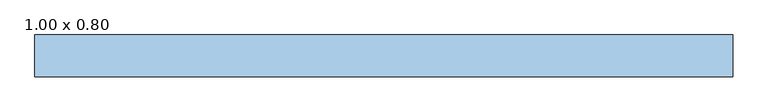
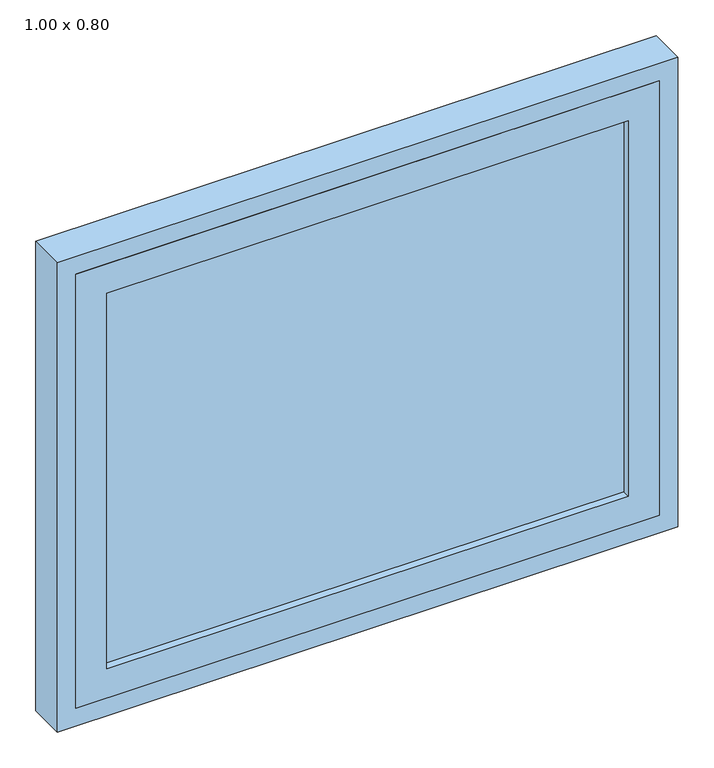
"""IFC4 building model written with IfcOpenShell, lengths in millimetres: window geometry, CC_JANELA MAXIM-AR_1 FOLHA VIDRO : 1.00 x 0.80."""

from ifc_helpers import new_model, si_unit, frame, origin, place, context, project, spatial, polyline, outline, extrude, source, transform, mapped, element, save


def window_1_00_x_0_80_3e14d2bc(model_context):
    return source(origin(), model_context, "Body", "SweptSolid", [
        extrude(outline(polyline([(-420.0, -87.5), (-420.0, -82.5), (420.0, -82.5), (420.0, -87.5), (-420.0, -87.5)])), frame((0.0, 0.0, 1780.0), z_axis=(0.0, 0.0, 1.0), x_axis=(1.0, 0.0, 0.0)), (0.0, 0.0, 1.0), 640.0),
        extrude(outline(polyline([(2470.0, -470.0), (1730.0, -470.0), (1730.0, 470.0), (2470.0, 470.0), (2470.0, -470.0)]), holes=[polyline([(2420.0, 420.0), (1780.0, 420.0), (1780.0, -420.0), (2420.0, -420.0), (2420.0, 420.0)])]), frame((0.0, -100.0, 0.0), z_axis=(0.0, 1.0, 0.0), x_axis=(0.0, 0.0, 1.0)), (0.0, 0.0, 1.0), 30.0),
        extrude(outline(polyline([(1700.0, 500.0), (2500.0, 500.0), (2500.0, -500.0), (1700.0, -500.0), (1700.0, 500.0)]), holes=[polyline([(1730.0, -470.0), (2470.0, -470.0), (2470.0, 470.0), (1730.0, 470.0), (1730.0, -470.0)])]), frame((0.0, -100.0, 0.0), z_axis=(0.0, 1.0, 0.0), x_axis=(0.0, 0.0, 1.0)), (0.0, 0.0, 1.0), 60.0),
    ])


if __name__ == "__main__":
    model = new_model("IFC4")
    model_context = context("Model", 3, world=origin())
    ifc_project = project(units=[si_unit("LENGTHUNIT", "METRE", prefix="MILLI")], contexts=[model_context])
    site = spatial("IfcSite", under=ifc_project)
    building = spatial("IfcBuilding", under=site)
    placement = place(None, origin())
    window_1_00_x_0_80_shape = window_1_00_x_0_80_3e14d2bc(model_context)
    element("IfcWindow", 1, ObjectType="CC_JANELA MAXIM-AR_1 FOLHA VIDRO : 1.00 x 0.80", at=placement, inside=building, context=model_context, shape_type="MappedRepresentation", body=[
        mapped(window_1_00_x_0_80_shape, transform((0.0, 0.0, 0.0), x_axis=(1.0, 0.0, 0.0), y_axis=(0.0, 1.0, 0.0), z_axis=(0.0, 0.0, 1.0))),
    ])
    save(model, "model.ifc")

# Revit data of these elements
# Type "CC_JANELA MAXIM-AR_1 FOLHA VIDRO : 1.00 x 0.80"
#   Type Mark = "J10"
#   Site = "www.construir.arq.br"
#   Empresa = "Cursos Construir"
#   Description = "JANELA MAXIM-AR 1 FOLHA VIDRO"
#   Criado Por = "Roberto Netto"
#   Analytic Construction = "<Nenhum>"
#   Atualizado por = "Rudemberg Eloi"
#   Rough Width = 1.00 m
#   Largura Moldura Folha [instance default] = 0.05 m
#   Largura Moldura Externa [instance default] = 0.10 m
#   Largura Guarnição Interna [instance default] = 0.05 m
#   Largura Folha [instance default] = 0.94 m
#   Interna [instance default] = 0.00 m
#   Externa [instance default] = 0.00 m
#   Extensão Frontal Peitoril/Pngadeira [instance default] = 0.03 m
#   Extensão Exterior Direita Peitoril/Pingadeira [instance default] = 0.025 m
#   Extensão Caixilho [instance default] = 0.03 m
#   Extensâo Exterior Esquerda Peitoril/Pingadeira [instance default] = 0.025 m
#   Espessura Peitoril/Pingadeira [instance default] = 0.02 m
#   Espessura Moldura Externa [instance default] = 0.01 m
#   Espessura Guarnição Interna [instance default] = 0.005 m
#   Espessura Folha [instance default] = 0.03 m
#   Espessura Caixilho [instance default] = 0.03 m
#   Cálculo Abertura Linear [instance default] = 0.00 m
#   Rough Height = 0.80 m
#   Altura Folha [instance default] = 0.74 m
#   Altura Corte [instance default] = 0.02 m
#   Height = 0.80 m
#   Width = 1.00 m
#   ----PEITORIL/PINGADEIRA---- [instance default] = 0.00 m
#   ----MOLDURA---- [instance default] = 0.00 m
#   ----GUARNIÇÃO---- [instance default] = 0.00 m
#   ----FOLHA---- [instance default] = 0.00 m
#   ----EXTENSÃO---- [instance default] = 0.00 m
#   ----CAIXILHO---- [instance default] = 0.00 m
#   Peitoril/Pingadeira Vazio [instance default] = no
#   Peitoril/Pingadeira Família [instance default] = yes
#   Moldura Externa [instance default] = no
#   Guarnição Interna [instance default] = yes
#   Material Vidro Folha = .VIDRO
#   Material Peitoril/Pingadeira = .GRANITO BRANCO ITAÚNAS
#   Material Moldura Folha = .ALUMÍNIO COM PINTURA ELETROSTÁTICA BRANCA
#   Material Moldura Externa = .PINTURA ACRÍLICA BRANCA
#   Material Guarnição = .ALUMÍNIO COM PINTURA ELETROSTÁTICA BRANCA
#   Material Caixilho = .ALUMÍNIO COM PINTURA ELETROSTÁTICA BRANCA
#   Wall Closure = (empty or 0)
# Element 1 (IfcWindow, "CC_JANELA MAXIM-AR_1 FOLHA VIDRO : 1.00 x 0.80")
#   Guarnição Interna = no
#   Materials on its faces: ".ALUMÍNIO COM PINTURA ELETROSTÁTICA BRANCA", ".VIDRO"
# Materials
#   ".VIDRO": class "Genérico", colour RGB 198 236 255, transparency 0.95, Cost = 0
#   ".GRANITO BRANCO ITAÚNAS": class ".CC_PEDRA REVEST.", colour RGB 202 195 174, transparency 0, Description = "Granito branco Itaúnas", Uso = "Pedra", Cost = 0
#   ".ALUMÍNIO COM PINTURA ELETROSTÁTICA BRANCA": class "CC_METAIS", colour RGB 241 241 241, transparency 0, Cost = 0
#   ".PINTURA ACRÍLICA BRANCA": class ".CC_PINTURA", colour RGB 250 250 250, transparency 0, Keynote = "09910.A1", Description = "Tinta acrílica na cor branca", Uso = "Pint.", Cost = 0
